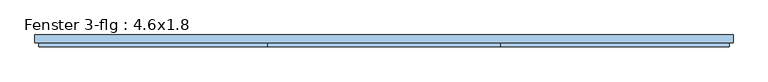
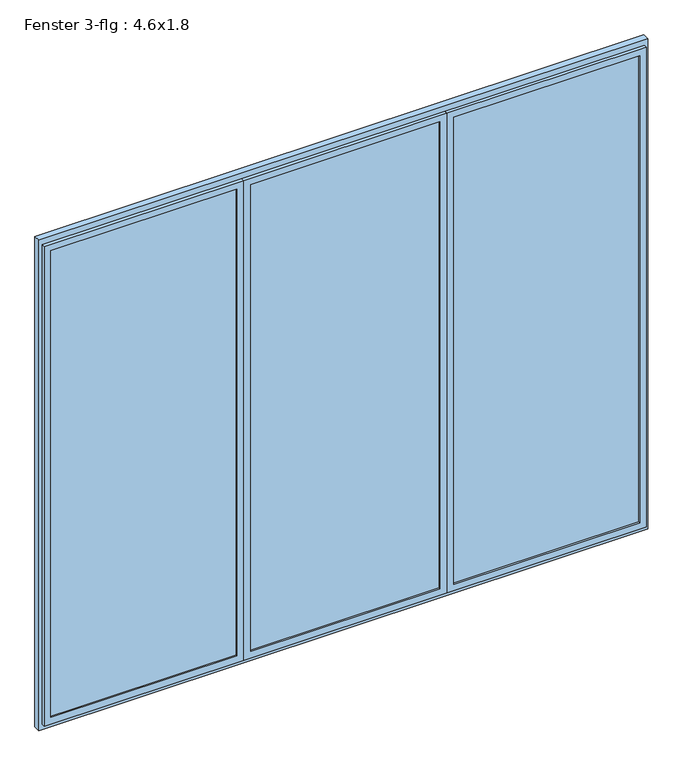
"""IFC4 building model written with IfcOpenShell, lengths in millimetres: window geometry, Fenster 3-flg : 4.6x1.8."""

import ifcopenshell
import ifcopenshell.guid

model = None  # the IFC model being written
_history = None  # IfcOwnerHistory: only IFC2X3 demands one
_inside = {}  # id of a spatial element -> (the spatial element, [elements in it])
_under = {}  # id of a project, library or spatial element -> (it, [spatial elements below it])
_declared = {}  # id of a project -> (the project, [libraries it declares])
_typed = {}  # id of a type object -> (the type object, [elements of that type])
_made_of = {}  # id of a material, layer set ... -> (it, [elements and type objects made of it])


def new_model(schema):
    """Start an empty IFC model of exactly this schema.

    Asked for "IFC4X3", IfcOpenShell would pick the latest addendum, in which some entities
    have other attributes; the version numbers below select the first issue.
    IFC2X3 requires an IfcOwnerHistory on every rooted entity: one is made here for all.
    """
    global model, _history
    if schema == "IFC4X3":
        model = ifcopenshell.file(schema_version=(4, 3, 0, 0))
    else:
        model = ifcopenshell.file(schema=schema)
    _inside.clear()
    _under.clear()
    _declared.clear()
    _typed.clear()
    _made_of.clear()
    _history = None
    if model.schema == "IFC2X3":
        org = make("IfcOrganization", Name="unknown")
        user = make(
            "IfcPersonAndOrganization",
            ThePerson=make("IfcPerson", FamilyName="unknown"),
            TheOrganization=org,
        )
        app = make(
            "IfcApplication",
            ApplicationDeveloper=org,
            Version="unknown",
            ApplicationFullName="unknown",
            ApplicationIdentifier="unknown",
        )
        _history = make(
            "IfcOwnerHistory",
            OwningUser=user,
            OwningApplication=app,
            ChangeAction="ADDED",
            CreationDate=0,
        )
    return model


def make(cls, **values):
    """One entity of the class cls with the attributes given. An attribute that is None is left unset."""
    return model.create_entity(
        cls, **{name: value for name, value in values.items() if value is not None}
    )


def rooted(cls, **values):
    """An entity with a GlobalId (a new one), such as an element, a storey or a relation."""
    return make(cls, GlobalId=ifcopenshell.guid.new(), OwnerHistory=_history, **values)


def si_unit(unit_type, name, prefix=None):
    """IfcSIUnit, for example si_unit("LENGTHUNIT", "METRE", prefix="MILLI")."""
    return make("IfcSIUnit", UnitType=unit_type, Prefix=prefix, Name=name)


def assignment(units):
    """IfcUnitAssignment: the units of a project."""
    return None if units is None else make("IfcUnitAssignment", Units=units)


def point(xyz):
    """IfcCartesianPoint."""
    return None if xyz is None else make("IfcCartesianPoint", Coordinates=xyz)


def direction(xyz):
    """IfcDirection."""
    return None if xyz is None else make("IfcDirection", DirectionRatios=xyz)


def frame(location, z_axis=None, x_axis=None):
    """IfcAxis2Placement3D, a coordinate frame: its origin and axes. An axis left out is left unset."""
    return make(
        "IfcAxis2Placement3D",
        Location=point(location),
        Axis=direction(z_axis),
        RefDirection=direction(x_axis),
    )


def origin():
    """The frame at (0, 0, 0) with its axes left unset."""
    return frame((0.0, 0.0, 0.0))


def place(relative_to, where):
    """IfcLocalPlacement: puts the frame where relative to a parent placement (None: the world)."""
    return make(
        "IfcLocalPlacement", PlacementRelTo=relative_to, RelativePlacement=where
    )


def context(
    kind, dimensions, precision=None, world=None, true_north=None, identifier=None
):
    """IfcGeometricRepresentationContext, for example the 3D "Model" context."""
    return make(
        "IfcGeometricRepresentationContext",
        ContextIdentifier=identifier,
        ContextType=kind,
        CoordinateSpaceDimension=dimensions,
        Precision=precision,
        WorldCoordinateSystem=world,
        TrueNorth=true_north,
    )


def project(units=None, contexts=None):
    """IfcProject with its units and contexts."""
    return rooted(
        "IfcProject",
        Name="project",
        RepresentationContexts=contexts,
        UnitsInContext=assignment(units),
    )


def spatial(cls, under=None, at=None, **own):
    """A site, building, storey or space (cls), placed at a placement, below another one or the project."""
    s = rooted(cls, ObjectPlacement=at, **own)
    if under is not None:
        _under.setdefault(under.id(), (under, []))[1].append(s)
    return s


def polyline(points):
    """IfcPolyline through the points."""
    return make("IfcPolyline", Points=[point(p) for p in points])


def outline(outer, holes=None, kind="AREA"):
    """IfcArbitraryClosedProfileDef: a profile drawn as a closed curve; with holes, ...WithVoids."""
    if holes is None:
        return make("IfcArbitraryClosedProfileDef", ProfileType=kind, OuterCurve=outer)
    return make(
        "IfcArbitraryProfileDefWithVoids",
        ProfileType=kind,
        OuterCurve=outer,
        InnerCurves=holes,
    )


def extrude(swept, where, along, depth):
    """IfcExtrudedAreaSolid: the profile swept, set in the frame where, extruded along a direction by depth."""
    return make(
        "IfcExtrudedAreaSolid",
        SweptArea=swept,
        Position=where,
        ExtrudedDirection=direction(along),
        Depth=depth,
    )


def faces_of(points, faces, orient=None, outer=None):
    """IfcFace entities. A face is a list of loops; a loop is a list of indices into points, from 0.

    orient and outer hold one flag for each loop. By default every Orientation is true, the
    first loop of a face is its IfcFaceOuterBound and the others are IfcFaceBound.
    """
    made = []
    for i, loops in enumerate(faces):
        bounds = []
        for j, loop in enumerate(loops):
            is_outer = j == 0 if outer is None else outer[i][j]
            bounds.append(
                make(
                    "IfcFaceOuterBound" if is_outer else "IfcFaceBound",
                    Bound=make("IfcPolyLoop", Polygon=[points[k] for k in loop]),
                    Orientation=True if orient is None else orient[i][j],
                )
            )
        made.append(make("IfcFace", Bounds=bounds))
    return made


def faceted_brep(points, faces, orient=None, outer=None, voids=None):
    """IfcFacetedBrep: a solid bounded by flat faces; with voids (closed shells), ...WithVoids."""
    shared = [point(p) for p in points]
    hull = make("IfcClosedShell", CfsFaces=faces_of(shared, faces, orient, outer))
    if voids is None:
        return make("IfcFacetedBrep", Outer=hull)
    return make(
        "IfcFacetedBrepWithVoids",
        Outer=hull,
        Voids=[
            make(cls, CfsFaces=faces_of(shared, fs, o, b)) for cls, fs, o, b in voids
        ],
    )


def shape(context_of_items, identifier, shape_type, items):
    """IfcShapeRepresentation: the items that make up one representation, for example the "Body"."""
    return make(
        "IfcShapeRepresentation",
        ContextOfItems=context_of_items,
        RepresentationIdentifier=identifier,
        RepresentationType=shape_type,
        Items=items,
    )


def source(mapping_origin, context_of_items, identifier, shape_type, items):
    """IfcRepresentationMap: a shape defined once, which mapped items show again and again."""
    return make(
        "IfcRepresentationMap",
        MappingOrigin=mapping_origin,
        MappedRepresentation=shape(context_of_items, identifier, shape_type, items),
    )


def transform(
    local_origin,
    x_axis=None,
    y_axis=None,
    z_axis=None,
    scale=None,
    scale2=None,
    scale3=None,
    uniform=True,
):
    """IfcCartesianTransformationOperator3D, or its non-uniform kind. x_axis, y_axis, z_axis: its Axis1, 2, 3."""
    if uniform:
        return make(
            "IfcCartesianTransformationOperator3D",
            Axis1=direction(x_axis),
            Axis2=direction(y_axis),
            LocalOrigin=point(local_origin),
            Scale=scale,
            Axis3=direction(z_axis),
        )
    return make(
        "IfcCartesianTransformationOperator3DnonUniform",
        Axis1=direction(x_axis),
        Axis2=direction(y_axis),
        LocalOrigin=point(local_origin),
        Scale=scale,
        Axis3=direction(z_axis),
        Scale2=scale2,
        Scale3=scale3,
    )


def mapped(mapping_source, mapping_target):
    """IfcMappedItem: shows the shape of a source again, moved by a transform."""
    return make(
        "IfcMappedItem", MappingSource=mapping_source, MappingTarget=mapping_target
    )


def made_of(thing, what):
    """Note that an element or type object is made of a material, layer set ...; save() writes the relation."""
    if what is not None:
        _made_of.setdefault(what.id(), (what, []))[1].append(thing)
    return thing


def element(
    cls,
    number,
    at=None,
    inside=None,
    cuts=None,
    type_object=None,
    material=None,
    context=None,
    identifier="Body",
    shape_type=None,
    held_by="IfcProductDefinitionShape",
    body=None,
    shapes=None,
    **own,
):
    """One element of the class cls, such as IfcWall. Its Tag is "e" and its number.

    at: its placement. inside: the storey or other place that contains it. cuts: it is an
    opening in that element (IfcRelVoidsElement). A single representation is given by context,
    identifier, shape_type and body (its items); several are given by shapes. held_by: the class
    of the entity that holds the representations. save() writes the other relations.
    """
    e = rooted(cls, Tag="e%d" % number, ObjectPlacement=at, **own)
    if body is not None:
        shapes = [shape(context, identifier, shape_type, body)]
    if shapes is not None:
        e.Representation = make(held_by, Representations=shapes)
    if inside is not None:
        _inside.setdefault(inside.id(), (inside, []))[1].append(e)
    if cuts is not None:
        rooted(
            "IfcRelVoidsElement", RelatingBuildingElement=cuts, RelatedOpeningElement=e
        )
    if type_object is not None:
        _typed.setdefault(type_object.id(), (type_object, []))[1].append(e)
    return made_of(e, material)


def aggregate(whole, parts):
    """IfcRelAggregates: a whole, such as a stair, and the parts it consists of."""
    return rooted("IfcRelAggregates", RelatingObject=whole, RelatedObjects=parts)


def save(model, path):
    """Write the relations noted so far, then the file.

    IfcRelAggregates (storeys below a building ...), IfcRelContainedInSpatialStructure (elements
    in a storey), IfcRelDefinesByType, IfcRelAssociatesMaterial and IfcRelDeclares: one each for
    every whole, place, type object, material and project.
    """
    for whole, parts in _under.values():
        aggregate(whole, parts)
    for where, things in _inside.values():
        rooted(
            "IfcRelContainedInSpatialStructure",
            RelatedElements=things,
            RelatingStructure=where,
        )
    for kind, things in _typed.values():
        rooted("IfcRelDefinesByType", RelatedObjects=things, RelatingType=kind)
    for what, things in _made_of.values():
        rooted("IfcRelAssociatesMaterial", RelatedObjects=things, RelatingMaterial=what)
    for by, libraries in _declared.values():
        rooted("IfcRelDeclares", RelatingContext=by, RelatedDefinitions=libraries)
    model.write(path)


def fenster_3_flg_4_6x1_8_bc6b32a3(model_context):
    return source(origin(), model_context, "Body", "SolidModel", [
        extrude(outline(polyline([(2500.0, 80.0), (2500.0, 20.0), (2440.0, 20.0), (2440.0, 80.0), (2500.0, 80.0)])), frame((0.0, 0.0, 1080.0), z_axis=(0.0, 0.0, 1.0), x_axis=(1.0, 0.0, 0.0)), (0.0, 0.0, 1.0), 4440.0),
        extrude(outline(polyline([(700.0, 80.0), (700.0, 20.0), (640.0, 20.0), (640.0, 80.0), (700.0, 80.0)])), frame((0.0, 0.0, 1080.0), z_axis=(0.0, 0.0, 1.0), x_axis=(1.0, 0.0, 0.0)), (0.0, 0.0, 1.0), 4440.0),
        extrude(outline(polyline([(5600.0, 4270.0), (5600.0, -1130.0), (1000.0, -1130.0), (1000.0, 4270.0), (5600.0, 4270.0)]), holes=[polyline([(5520.0, 4210.0), (1080.0, 4210.0), (1080.0, -1070.0), (5520.0, -1070.0), (5520.0, 4210.0)])]), frame((0.0, 20.0, 0.0), z_axis=(0.0, 1.0, 0.0), x_axis=(0.0, 0.0, 1.0)), (0.0, 0.0, 1.0), 60.0),
        faceted_brep([(2470.0, 20.0, 5550.0), (2470.0, -10.0, 5550.0), (2470.0, -10.0, 1050.0), (2470.0, 20.0, 1050.0), (670.0, -10.0, 5550.0), (670.0, -10.0, 1050.0), (2410.0, -10.0, 1110.0), (730.0, -10.0, 1110.0), (730.0, -10.0, 5490.0), (2410.0, -10.0, 5490.0), (670.0, 20.0, 1050.0), (670.0, 20.0, 5550.0), (2440.0, 20.0, 5520.0), (700.0, 20.0, 5520.0), (700.0, 20.0, 1080.0), (2440.0, 20.0, 1080.0), (2440.0, 50.0, 5520.0), (2440.0, 50.0, 1080.0), (700.0, 50.0, 1080.0), (700.0, 50.0, 5520.0), (2410.0, 50.0, 5490.0), (730.0, 50.0, 5490.0), (730.0, 50.0, 1110.0), (2410.0, 50.0, 1110.0)], [[[0, 1, 2, 3]], [[1, 4, 5, 2], [6, 7, 8, 9]], [[3, 2, 5, 10]], [[3, 10, 11, 0], [12, 13, 14, 15]], [[16, 12, 15, 17]], [[17, 15, 14, 18]], [[17, 18, 19, 16], [20, 21, 22, 23]], [[9, 20, 23, 6]], [[6, 23, 22, 7]], [[10, 5, 4, 11]], [[18, 14, 13, 19]], [[7, 22, 21, 8]], [[11, 4, 1, 0]], [[19, 13, 12, 16]], [[8, 21, 20, 9]]]),
        faceted_brep([(670.0, 20.0, 5550.0), (670.0, -10.0, 5550.0), (670.0, -10.0, 1050.0), (670.0, 20.0, 1050.0), (-1100.0, -10.0, 5550.0), (-1100.0, -10.0, 1050.0), (610.0, -10.0, 1110.0), (-1040.0, -10.0, 1110.0), (-1040.0, -10.0, 5490.0), (610.0, -10.0, 5490.0), (-1100.0, 20.0, 1050.0), (-1100.0, 20.0, 5550.0), (640.0, 20.0, 5520.0), (-1070.0, 20.0, 5520.0), (-1070.0, 20.0, 1080.0), (640.0, 20.0, 1080.0), (640.0, 50.0, 5520.0), (640.0, 50.0, 1080.0), (-1070.0, 50.0, 1080.0), (-1070.0, 50.0, 5520.0), (610.0, 50.0, 5490.0), (-1040.0, 50.0, 5490.0), (-1040.0, 50.0, 1110.0), (610.0, 50.0, 1110.0)], [[[0, 1, 2, 3]], [[1, 4, 5, 2], [6, 7, 8, 9]], [[3, 2, 5, 10]], [[3, 10, 11, 0], [12, 13, 14, 15]], [[16, 12, 15, 17]], [[17, 15, 14, 18]], [[17, 18, 19, 16], [20, 21, 22, 23]], [[9, 20, 23, 6]], [[6, 23, 22, 7]], [[10, 5, 4, 11]], [[18, 14, 13, 19]], [[7, 22, 21, 8]], [[11, 4, 1, 0]], [[19, 13, 12, 16]], [[8, 21, 20, 9]]]),
        faceted_brep([(4240.0, 20.0, 5550.0), (4240.0, -10.0, 5550.0), (4240.0, -10.0, 1050.0), (4240.0, 20.0, 1050.0), (2470.0, -10.0, 5550.0), (2470.0, -10.0, 1050.0), (4180.0, -10.0, 1110.0), (2530.0, -10.0, 1110.0), (2530.0, -10.0, 5490.0), (4180.0, -10.0, 5490.0), (2470.0, 20.0, 1050.0), (2470.0, 20.0, 5550.0), (4210.0, 20.0, 5520.0), (2500.0, 20.0, 5520.0), (2500.0, 20.0, 1080.0), (4210.0, 20.0, 1080.0), (4210.0, 50.0, 5520.0), (4210.0, 50.0, 1080.0), (2500.0, 50.0, 1080.0), (2500.0, 50.0, 5520.0), (4180.0, 50.0, 5490.0), (2530.0, 50.0, 5490.0), (2530.0, 50.0, 1110.0), (4180.0, 50.0, 1110.0)], [[[0, 1, 2, 3]], [[1, 4, 5, 2], [6, 7, 8, 9]], [[3, 2, 5, 10]], [[3, 10, 11, 0], [12, 13, 14, 15]], [[16, 12, 15, 17]], [[17, 15, 14, 18]], [[17, 18, 19, 16], [20, 21, 22, 23]], [[9, 20, 23, 6]], [[6, 23, 22, 7]], [[10, 5, 4, 11]], [[18, 14, 13, 19]], [[7, 22, 21, 8]], [[11, 4, 1, 0]], [[19, 13, 12, 16]], [[8, 21, 20, 9]]]),
        extrude(outline(polyline([(4180.0, 5.0), (2530.0, 5.0), (2530.0, 35.0), (4180.0, 35.0), (4180.0, 5.0)])), frame((0.0, 0.0, 1110.0), z_axis=(0.0, 0.0, 1.0), x_axis=(1.0, 0.0, 0.0)), (0.0, 0.0, 1.0), 4380.0),
        extrude(outline(polyline([(2410.0, 5.0), (730.0, 5.0), (730.0, 35.0), (2410.0, 35.0), (2410.0, 5.0)])), frame((0.0, 0.0, 1110.0), z_axis=(0.0, 0.0, 1.0), x_axis=(1.0, 0.0, 0.0)), (0.0, 0.0, 1.0), 4380.0),
        extrude(outline(polyline([(610.0, 5.0), (-1040.0, 5.0), (-1040.0, 35.0), (610.0, 35.0), (610.0, 5.0)])), frame((0.0, 0.0, 1110.0), z_axis=(0.0, 0.0, 1.0), x_axis=(1.0, 0.0, 0.0)), (0.0, 0.0, 1.0), 4380.0),
    ])


if __name__ == "__main__":
    model = new_model("IFC4")
    model_context = context("Model", 3, world=origin())
    ifc_project = project(units=[si_unit("LENGTHUNIT", "METRE", prefix="MILLI")], contexts=[model_context])
    site = spatial("IfcSite", under=ifc_project)
    building = spatial("IfcBuilding", under=site)
    placement = place(None, origin())
    fenster_3_flg_4_6x1_8_shape = fenster_3_flg_4_6x1_8_bc6b32a3(model_context)
    element("IfcWindow", 1, ObjectType="Fenster 3-flg : 4.6x1.8", at=placement, inside=building, context=model_context, shape_type="MappedRepresentation", body=[
        mapped(fenster_3_flg_4_6x1_8_shape, transform((0.0, 0.0, 0.0), x_axis=(1.0, 0.0, 0.0), y_axis=(0.0, 1.0, 0.0), z_axis=(0.0, 0.0, 1.0))),
    ])
    save(model, "model.ifc")

# Revit data of these elements
# Type "Fenster 3-flg : 4.6x1.8"
#   Type Mark = "63"
#   Operation = "TriplePanelVertical"
#   Keynote = "16.05.01"
#   Visual Light Transmittance = 0.9
#   Solar Heat Gain Coefficient = 0.78
#   Rough Height = 4.600 m
#   Rough Width = 5.400 m
#   Heat Transfer Coefficient (U) = 3.6886 W/(m²·K)
#   Rahmentiefe = 0.060 m
#   Breite unterer Rahmen = 0.080 m
#   Breite oberer  Rahmen = 0.080 m
#   Rahmenbreite = 0.060 m
#   Height = 4.600 m
#   Tiefe Flügel = 0.060 m
#   Flügelbreite = 0.060 m
#   Einbautiefe (von außen) [instance default] = 0.080 m
#   Width = 5.400 m
#   Bild [instance default] = none
#   Glas [instance default] = none
#   Fensterflügel [instance default] = none
#   Innere Fensterbank [instance default] = none
#   Äußere Fensterbank [instance default] = none
#   Construction Type Id = ""
#   Wall Closure = (empty or 0)
#   Analytic Construction = (empty or 0)
# Element 1 (IfcWindow, "Fenster 3-flg : 4.6x1.8")
#   Einbautiefe (von außen) = 0.230 m
#   Materials on its faces: "Kunststoff - Weiß", "Glas"
# Materials
#   "Kunststoff - Weiß": class "Kunststoff", colour RGB 249 249 249, transparency 0, Cost = 0
#   "Glas": class "Glas", colour RGB 0 0 255, transparency 0.75, Comments = "Render-Darstellung nicht aktualisiert ", Cost = 0
